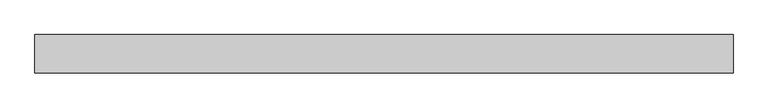
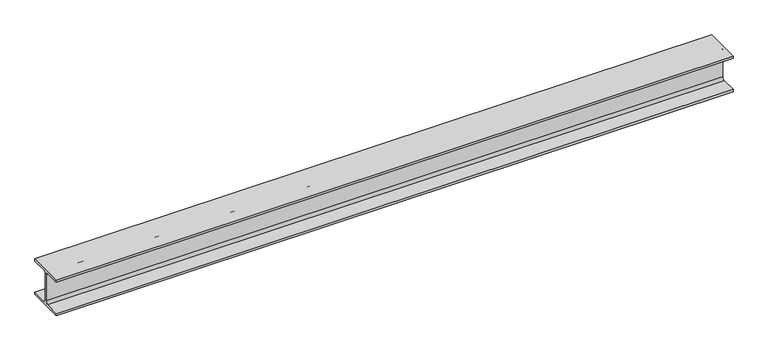
"""IFC4 building model written with IfcOpenShell, lengths in millimetres: beam geometry, 0912_Steel Framing_H-KSD3502 : H_SB_ASB_H-200x200x8x12."""

import ifcopenshell
import ifcopenshell.guid

model = None  # the IFC model being written
_history = None  # IfcOwnerHistory: only IFC2X3 demands one
_inside = {}  # id of a spatial element -> (the spatial element, [elements in it])
_under = {}  # id of a project, library or spatial element -> (it, [spatial elements below it])
_declared = {}  # id of a project -> (the project, [libraries it declares])
_typed = {}  # id of a type object -> (the type object, [elements of that type])
_made_of = {}  # id of a material, layer set ... -> (it, [elements and type objects made of it])


def new_model(schema):
    """Start an empty IFC model of exactly this schema.

    Asked for "IFC4X3", IfcOpenShell would pick the latest addendum, in which some entities
    have other attributes; the version numbers below select the first issue.
    IFC2X3 requires an IfcOwnerHistory on every rooted entity: one is made here for all.
    """
    global model, _history
    if schema == "IFC4X3":
        model = ifcopenshell.file(schema_version=(4, 3, 0, 0))
    else:
        model = ifcopenshell.file(schema=schema)
    _inside.clear()
    _under.clear()
    _declared.clear()
    _typed.clear()
    _made_of.clear()
    _history = None
    if model.schema == "IFC2X3":
        org = make("IfcOrganization", Name="unknown")
        user = make(
            "IfcPersonAndOrganization",
            ThePerson=make("IfcPerson", FamilyName="unknown"),
            TheOrganization=org,
        )
        app = make(
            "IfcApplication",
            ApplicationDeveloper=org,
            Version="unknown",
            ApplicationFullName="unknown",
            ApplicationIdentifier="unknown",
        )
        _history = make(
            "IfcOwnerHistory",
            OwningUser=user,
            OwningApplication=app,
            ChangeAction="ADDED",
            CreationDate=0,
        )
    return model


def make(cls, **values):
    """One entity of the class cls with the attributes given. An attribute that is None is left unset."""
    return model.create_entity(
        cls, **{name: value for name, value in values.items() if value is not None}
    )


def rooted(cls, **values):
    """An entity with a GlobalId (a new one), such as an element, a storey or a relation."""
    return make(cls, GlobalId=ifcopenshell.guid.new(), OwnerHistory=_history, **values)


def si_unit(unit_type, name, prefix=None):
    """IfcSIUnit, for example si_unit("LENGTHUNIT", "METRE", prefix="MILLI")."""
    return make("IfcSIUnit", UnitType=unit_type, Prefix=prefix, Name=name)


def assignment(units):
    """IfcUnitAssignment: the units of a project."""
    return None if units is None else make("IfcUnitAssignment", Units=units)


def point(xyz):
    """IfcCartesianPoint."""
    return None if xyz is None else make("IfcCartesianPoint", Coordinates=xyz)


def direction(xyz):
    """IfcDirection."""
    return None if xyz is None else make("IfcDirection", DirectionRatios=xyz)


def frame(location, z_axis=None, x_axis=None):
    """IfcAxis2Placement3D, a coordinate frame: its origin and axes. An axis left out is left unset."""
    return make(
        "IfcAxis2Placement3D",
        Location=point(location),
        Axis=direction(z_axis),
        RefDirection=direction(x_axis),
    )


def frame_2d(location, x_axis=None):
    """IfcAxis2Placement2D, a coordinate frame in the plane: its origin and x axis."""
    return make(
        "IfcAxis2Placement2D", Location=point(location), RefDirection=direction(x_axis)
    )


def origin():
    """The frame at (0, 0, 0) with its axes left unset."""
    return frame((0.0, 0.0, 0.0))


def place(relative_to, where):
    """IfcLocalPlacement: puts the frame where relative to a parent placement (None: the world)."""
    return make(
        "IfcLocalPlacement", PlacementRelTo=relative_to, RelativePlacement=where
    )


def context(
    kind, dimensions, precision=None, world=None, true_north=None, identifier=None
):
    """IfcGeometricRepresentationContext, for example the 3D "Model" context."""
    return make(
        "IfcGeometricRepresentationContext",
        ContextIdentifier=identifier,
        ContextType=kind,
        CoordinateSpaceDimension=dimensions,
        Precision=precision,
        WorldCoordinateSystem=world,
        TrueNorth=true_north,
    )


def project(units=None, contexts=None):
    """IfcProject with its units and contexts."""
    return rooted(
        "IfcProject",
        Name="project",
        RepresentationContexts=contexts,
        UnitsInContext=assignment(units),
    )


def spatial(cls, under=None, at=None, **own):
    """A site, building, storey or space (cls), placed at a placement, below another one or the project."""
    s = rooted(cls, ObjectPlacement=at, **own)
    if under is not None:
        _under.setdefault(under.id(), (under, []))[1].append(s)
    return s


def polyline(points):
    """IfcPolyline through the points."""
    return make("IfcPolyline", Points=[point(p) for p in points])


def circle_curve(where, radius):
    """IfcCircle in the frame where."""
    return make("IfcCircle", Position=where, Radius=radius)


def trimmed(basis, trim1, trim2, sense, master):
    """IfcTrimmedCurve: the piece of a basis curve between two trims."""
    return make(
        "IfcTrimmedCurve",
        BasisCurve=basis,
        Trim1=trim1,
        Trim2=trim2,
        SenseAgreement=sense,
        MasterRepresentation=master,
    )


def segment(curve, same_sense, transition):
    """IfcCompositeCurveSegment."""
    return make(
        "IfcCompositeCurveSegment",
        Transition=transition,
        SameSense=same_sense,
        ParentCurve=curve,
    )


def composite_curve(segments, self_intersect=None):
    """IfcCompositeCurve: segments joined end to end."""
    return make("IfcCompositeCurve", Segments=segments, SelfIntersect=self_intersect)


def outline(outer, holes=None, kind="AREA"):
    """IfcArbitraryClosedProfileDef: a profile drawn as a closed curve; with holes, ...WithVoids."""
    if holes is None:
        return make("IfcArbitraryClosedProfileDef", ProfileType=kind, OuterCurve=outer)
    return make(
        "IfcArbitraryProfileDefWithVoids",
        ProfileType=kind,
        OuterCurve=outer,
        InnerCurves=holes,
    )


def extrude(swept, where, along, depth):
    """IfcExtrudedAreaSolid: the profile swept, set in the frame where, extruded along a direction by depth."""
    return make(
        "IfcExtrudedAreaSolid",
        SweptArea=swept,
        Position=where,
        ExtrudedDirection=direction(along),
        Depth=depth,
    )


def shape(context_of_items, identifier, shape_type, items):
    """IfcShapeRepresentation: the items that make up one representation, for example the "Body"."""
    return make(
        "IfcShapeRepresentation",
        ContextOfItems=context_of_items,
        RepresentationIdentifier=identifier,
        RepresentationType=shape_type,
        Items=items,
    )


def source(mapping_origin, context_of_items, identifier, shape_type, items):
    """IfcRepresentationMap: a shape defined once, which mapped items show again and again."""
    return make(
        "IfcRepresentationMap",
        MappingOrigin=mapping_origin,
        MappedRepresentation=shape(context_of_items, identifier, shape_type, items),
    )


def transform(
    local_origin,
    x_axis=None,
    y_axis=None,
    z_axis=None,
    scale=None,
    scale2=None,
    scale3=None,
    uniform=True,
):
    """IfcCartesianTransformationOperator3D, or its non-uniform kind. x_axis, y_axis, z_axis: its Axis1, 2, 3."""
    if uniform:
        return make(
            "IfcCartesianTransformationOperator3D",
            Axis1=direction(x_axis),
            Axis2=direction(y_axis),
            LocalOrigin=point(local_origin),
            Scale=scale,
            Axis3=direction(z_axis),
        )
    return make(
        "IfcCartesianTransformationOperator3DnonUniform",
        Axis1=direction(x_axis),
        Axis2=direction(y_axis),
        LocalOrigin=point(local_origin),
        Scale=scale,
        Axis3=direction(z_axis),
        Scale2=scale2,
        Scale3=scale3,
    )


def mapped(mapping_source, mapping_target):
    """IfcMappedItem: shows the shape of a source again, moved by a transform."""
    return make(
        "IfcMappedItem", MappingSource=mapping_source, MappingTarget=mapping_target
    )


def made_of(thing, what):
    """Note that an element or type object is made of a material, layer set ...; save() writes the relation."""
    if what is not None:
        _made_of.setdefault(what.id(), (what, []))[1].append(thing)
    return thing


def element(
    cls,
    number,
    at=None,
    inside=None,
    cuts=None,
    type_object=None,
    material=None,
    context=None,
    identifier="Body",
    shape_type=None,
    held_by="IfcProductDefinitionShape",
    body=None,
    shapes=None,
    **own,
):
    """One element of the class cls, such as IfcWall. Its Tag is "e" and its number.

    at: its placement. inside: the storey or other place that contains it. cuts: it is an
    opening in that element (IfcRelVoidsElement). A single representation is given by context,
    identifier, shape_type and body (its items); several are given by shapes. held_by: the class
    of the entity that holds the representations. save() writes the other relations.
    """
    e = rooted(cls, Tag="e%d" % number, ObjectPlacement=at, **own)
    if body is not None:
        shapes = [shape(context, identifier, shape_type, body)]
    if shapes is not None:
        e.Representation = make(held_by, Representations=shapes)
    if inside is not None:
        _inside.setdefault(inside.id(), (inside, []))[1].append(e)
    if cuts is not None:
        rooted(
            "IfcRelVoidsElement", RelatingBuildingElement=cuts, RelatedOpeningElement=e
        )
    if type_object is not None:
        _typed.setdefault(type_object.id(), (type_object, []))[1].append(e)
    return made_of(e, material)


def aggregate(whole, parts):
    """IfcRelAggregates: a whole, such as a stair, and the parts it consists of."""
    return rooted("IfcRelAggregates", RelatingObject=whole, RelatedObjects=parts)


def save(model, path):
    """Write the relations noted so far, then the file.

    IfcRelAggregates (storeys below a building ...), IfcRelContainedInSpatialStructure (elements
    in a storey), IfcRelDefinesByType, IfcRelAssociatesMaterial and IfcRelDeclares: one each for
    every whole, place, type object, material and project.
    """
    for whole, parts in _under.values():
        aggregate(whole, parts)
    for where, things in _inside.values():
        rooted(
            "IfcRelContainedInSpatialStructure",
            RelatedElements=things,
            RelatingStructure=where,
        )
    for kind, things in _typed.values():
        rooted("IfcRelDefinesByType", RelatedObjects=things, RelatingType=kind)
    for what, things in _made_of.values():
        rooted("IfcRelAssociatesMaterial", RelatedObjects=things, RelatingMaterial=what)
    for by, libraries in _declared.values():
        rooted("IfcRelDeclares", RelatingContext=by, RelatedDefinitions=libraries)
    model.write(path)


def beam_006f807e(model_context):
    return source(origin(), model_context, "Body", "SweptSolid", [
        extrude(outline(composite_curve([segment(polyline([(-100.0, -88.0), (-17.0, -88.0)]), True, "CONTINUOUS"), segment(trimmed(circle_curve(frame_2d((-17.0, -75.0)), 13.0), [point((-17.0, -88.0))], [point((-4.0, -75.0))], True, "CARTESIAN"), True, "CONTINUOUS"), segment(polyline([(-4.0, -75.0), (-4.0, 75.0)]), True, "CONTINUOUS"), segment(trimmed(circle_curve(frame_2d((-17.0, 75.0)), 13.0), [point((-4.0, 75.0))], [point((-17.0, 88.0))], True, "CARTESIAN"), True, "CONTINUOUS"), segment(polyline([(-17.0, 88.0), (-100.0, 88.0), (-100.0, 100.0), (100.0, 100.0), (100.0, 88.0), (17.0, 88.0)]), True, "CONTINUOUS"), segment(trimmed(circle_curve(frame_2d((17.0, 75.0)), 13.0), [point((17.0, 88.0))], [point((4.0, 75.0))], True, "CARTESIAN"), True, "CONTINUOUS"), segment(polyline([(4.0, 75.0), (4.0, -75.0)]), True, "CONTINUOUS"), segment(trimmed(circle_curve(frame_2d((17.0, -75.0)), 13.0), [point((4.0, -75.0))], [point((17.0, -88.0))], True, "CARTESIAN"), True, "CONTINUOUS"), segment(polyline([(17.0, -88.0), (100.0, -88.0), (100.0, -100.0), (-100.0, -100.0), (-100.0, -88.0)]), True, "CONTINUOUS")], self_intersect=False)), frame((-1827.2740995, 0.0, 0.0), z_axis=(1.0, 0.0, 0.0), x_axis=(0.0, 1.0, 0.0)), (0.0, 0.0, 1.0), 3629.4587666),
    ])


if __name__ == "__main__":
    model = new_model("IFC4")
    model_context = context("Model", 3, world=origin())
    ifc_project = project(units=[si_unit("LENGTHUNIT", "METRE", prefix="MILLI")], contexts=[model_context])
    site = spatial("IfcSite", under=ifc_project)
    building = spatial("IfcBuilding", under=site)
    placement = place(None, origin())
    beam_shape = beam_006f807e(model_context)
    element("IfcBeam", 1, ObjectType="0912_Steel Framing_H-KSD3502 : H_SB_ASB_H-200x200x8x12", at=placement, inside=building, context=model_context, shape_type="MappedRepresentation", body=[
        mapped(beam_shape, transform((0.0, 0.0, 0.0), x_axis=(1.0, 0.0, 0.0), y_axis=(0.0, 1.0, 0.0), z_axis=(0.0, 0.0, 1.0))),
    ])
    save(model, "model.ifc")

# Revit data of these elements
# Project information
#   Building Name = "STEAM TURBINE BUILDING"
#   H_Building Tag = "STB"
#   Project Status = "종결"
#   Client Name = "Therma Viayas Inc.\nTherma Viayas Inc.\nTherma Viayas Inc.\nTherma Viayas Inc."
#   Project Name = "Therma Visayas 2*150MW CFB Power Plant"
#   Project Number = "BEPH1402"
# Type "0912_Steel Framing_H-KSD3502 : H_SB_ASB_H-200x200x8x12"
#   H_WM Code_1 = "S01AA002-00001 | Main Steel Structure Fabrication Work | Shelter/Building | Medium Steel - Standard (90KG/M>Weight≥30KG/M) | Material: (   )"
#   H_WM Code_2 = "S03AA028-00001 | Main Steel Structure Erection Work | Shelter/Building | Medium Steel (90KG/M>Weight≥30KG/M) | Material: (   )"
#   H_WM Code_3 = "S01AA010-00001 | Main Steel Structure Fabrication Work | Shelter/Building | Steel Painting/Coating | for Non-Fireproofed Steel Surface, Surface Preparation, Primer, Second & Final Coat | Material: (   )"
#   H_Q'ty Cal Type Tag = "SB-Q2"
#   Width = 20.0 cm
#   Web Thickness = 0.8 cm
#   Web Fillet = 1.3 cm
#   Warping Constant = 141000.0 cm⁶
#   W = 0
#   Torsional Moment of Inertia = 26.2485 cm⁴
#   Section Area = 63.53 cm²
#   Plastic Modulus weak axis = 244.0 cm³
#   Plastic Modulus strong axis = 525.0 cm³
#   Perimeter = 1.16 m²/m
#   Nominal Weight = 49.90 kgf/m
#   Moment of Inertia weak axis = 1600.00 cm⁴
#   Moment of Inertia strong axis = 4720.00 cm⁴
#   Height = 20.0 cm
#   Flange Thickness = 1.2 cm
#   Elastic Modulus weak axis = 160.0 cm³
#   Elastic Modulus strong axis = 472.0 cm³
#   Centroid Vertical = 10.0 cm
#   Centroid Horizontal = 10.0 cm
#   Ix = 47200000
#   Length [instance default] = 1.5240 m
#   Zx = 525000
#   b = 0.2000 m
#   h = 0.2000 m
#   r = 0.0130 m
#   s = 0.0080 m
#   t = 0.0120 m
#   A = 0.006353 m²
#   Structural Material [instance default] = Steel, 45-345
#   Assembly Code = ""
# Element 1 (IfcBeam, "0912_Steel Framing_H-KSD3502 : H_SB_ASB_H-200x200x8x12")
#   Structural Material = none
# Materials
#   "Steel, 45-345": class "Metal", colour RGB 189 187 185, transparency 0, Description = "Steel 345 MPa", Cost = 0
